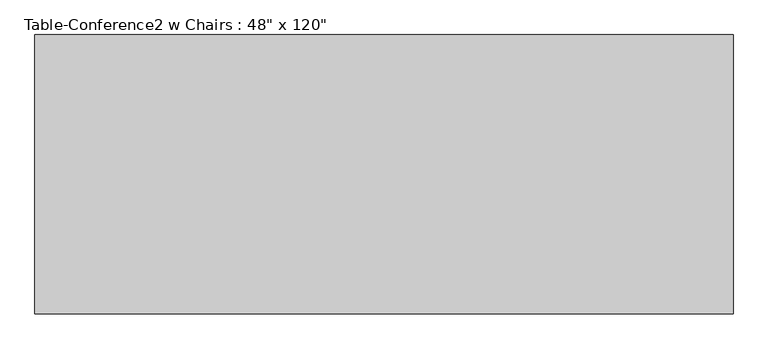
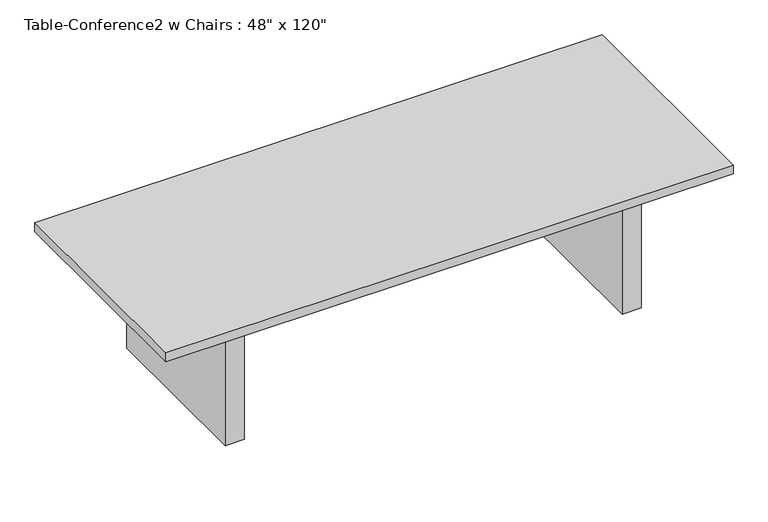
"""IFC4 building model written with IfcOpenShell, lengths in millimetres: furniture geometry."""

import ifcopenshell
import ifcopenshell.guid

model = None  # the IFC model being written
_history = None  # IfcOwnerHistory: only IFC2X3 demands one
_inside = {}  # id of a spatial element -> (the spatial element, [elements in it])
_under = {}  # id of a project, library or spatial element -> (it, [spatial elements below it])
_declared = {}  # id of a project -> (the project, [libraries it declares])
_typed = {}  # id of a type object -> (the type object, [elements of that type])
_made_of = {}  # id of a material, layer set ... -> (it, [elements and type objects made of it])


def new_model(schema):
    """Start an empty IFC model of exactly this schema.

    Asked for "IFC4X3", IfcOpenShell would pick the latest addendum, in which some entities
    have other attributes; the version numbers below select the first issue.
    IFC2X3 requires an IfcOwnerHistory on every rooted entity: one is made here for all.
    """
    global model, _history
    if schema == "IFC4X3":
        model = ifcopenshell.file(schema_version=(4, 3, 0, 0))
    else:
        model = ifcopenshell.file(schema=schema)
    _inside.clear()
    _under.clear()
    _declared.clear()
    _typed.clear()
    _made_of.clear()
    _history = None
    if model.schema == "IFC2X3":
        org = make("IfcOrganization", Name="unknown")
        user = make(
            "IfcPersonAndOrganization",
            ThePerson=make("IfcPerson", FamilyName="unknown"),
            TheOrganization=org,
        )
        app = make(
            "IfcApplication",
            ApplicationDeveloper=org,
            Version="unknown",
            ApplicationFullName="unknown",
            ApplicationIdentifier="unknown",
        )
        _history = make(
            "IfcOwnerHistory",
            OwningUser=user,
            OwningApplication=app,
            ChangeAction="ADDED",
            CreationDate=0,
        )
    return model


def make(cls, **values):
    """One entity of the class cls with the attributes given. An attribute that is None is left unset."""
    return model.create_entity(
        cls, **{name: value for name, value in values.items() if value is not None}
    )


def rooted(cls, **values):
    """An entity with a GlobalId (a new one), such as an element, a storey or a relation."""
    return make(cls, GlobalId=ifcopenshell.guid.new(), OwnerHistory=_history, **values)


def si_unit(unit_type, name, prefix=None):
    """IfcSIUnit, for example si_unit("LENGTHUNIT", "METRE", prefix="MILLI")."""
    return make("IfcSIUnit", UnitType=unit_type, Prefix=prefix, Name=name)


def assignment(units):
    """IfcUnitAssignment: the units of a project."""
    return None if units is None else make("IfcUnitAssignment", Units=units)


def point(xyz):
    """IfcCartesianPoint."""
    return None if xyz is None else make("IfcCartesianPoint", Coordinates=xyz)


def direction(xyz):
    """IfcDirection."""
    return None if xyz is None else make("IfcDirection", DirectionRatios=xyz)


def frame(location, z_axis=None, x_axis=None):
    """IfcAxis2Placement3D, a coordinate frame: its origin and axes. An axis left out is left unset."""
    return make(
        "IfcAxis2Placement3D",
        Location=point(location),
        Axis=direction(z_axis),
        RefDirection=direction(x_axis),
    )


def origin():
    """The frame at (0, 0, 0) with its axes left unset."""
    return frame((0.0, 0.0, 0.0))


def origin_with_axes():
    """The frame at (0, 0, 0) with the z axis (0, 0, 1) and the x axis (1, 0, 0) written out."""
    return frame((0.0, 0.0, 0.0), z_axis=(0.0, 0.0, 1.0), x_axis=(1.0, 0.0, 0.0))


def place(relative_to, where):
    """IfcLocalPlacement: puts the frame where relative to a parent placement (None: the world)."""
    return make(
        "IfcLocalPlacement", PlacementRelTo=relative_to, RelativePlacement=where
    )


def context(
    kind, dimensions, precision=None, world=None, true_north=None, identifier=None
):
    """IfcGeometricRepresentationContext, for example the 3D "Model" context."""
    return make(
        "IfcGeometricRepresentationContext",
        ContextIdentifier=identifier,
        ContextType=kind,
        CoordinateSpaceDimension=dimensions,
        Precision=precision,
        WorldCoordinateSystem=world,
        TrueNorth=true_north,
    )


def project(units=None, contexts=None):
    """IfcProject with its units and contexts."""
    return rooted(
        "IfcProject",
        Name="project",
        RepresentationContexts=contexts,
        UnitsInContext=assignment(units),
    )


def spatial(cls, under=None, at=None, **own):
    """A site, building, storey or space (cls), placed at a placement, below another one or the project."""
    s = rooted(cls, ObjectPlacement=at, **own)
    if under is not None:
        _under.setdefault(under.id(), (under, []))[1].append(s)
    return s


def polyline(points):
    """IfcPolyline through the points."""
    return make("IfcPolyline", Points=[point(p) for p in points])


def outline(outer, holes=None, kind="AREA"):
    """IfcArbitraryClosedProfileDef: a profile drawn as a closed curve; with holes, ...WithVoids."""
    if holes is None:
        return make("IfcArbitraryClosedProfileDef", ProfileType=kind, OuterCurve=outer)
    return make(
        "IfcArbitraryProfileDefWithVoids",
        ProfileType=kind,
        OuterCurve=outer,
        InnerCurves=holes,
    )


def extrude(swept, where, along, depth):
    """IfcExtrudedAreaSolid: the profile swept, set in the frame where, extruded along a direction by depth."""
    return make(
        "IfcExtrudedAreaSolid",
        SweptArea=swept,
        Position=where,
        ExtrudedDirection=direction(along),
        Depth=depth,
    )


def shape(context_of_items, identifier, shape_type, items):
    """IfcShapeRepresentation: the items that make up one representation, for example the "Body"."""
    return make(
        "IfcShapeRepresentation",
        ContextOfItems=context_of_items,
        RepresentationIdentifier=identifier,
        RepresentationType=shape_type,
        Items=items,
    )


def source(mapping_origin, context_of_items, identifier, shape_type, items):
    """IfcRepresentationMap: a shape defined once, which mapped items show again and again."""
    return make(
        "IfcRepresentationMap",
        MappingOrigin=mapping_origin,
        MappedRepresentation=shape(context_of_items, identifier, shape_type, items),
    )


def transform(
    local_origin,
    x_axis=None,
    y_axis=None,
    z_axis=None,
    scale=None,
    scale2=None,
    scale3=None,
    uniform=True,
):
    """IfcCartesianTransformationOperator3D, or its non-uniform kind. x_axis, y_axis, z_axis: its Axis1, 2, 3."""
    if uniform:
        return make(
            "IfcCartesianTransformationOperator3D",
            Axis1=direction(x_axis),
            Axis2=direction(y_axis),
            LocalOrigin=point(local_origin),
            Scale=scale,
            Axis3=direction(z_axis),
        )
    return make(
        "IfcCartesianTransformationOperator3DnonUniform",
        Axis1=direction(x_axis),
        Axis2=direction(y_axis),
        LocalOrigin=point(local_origin),
        Scale=scale,
        Axis3=direction(z_axis),
        Scale2=scale2,
        Scale3=scale3,
    )


def mapped(mapping_source, mapping_target):
    """IfcMappedItem: shows the shape of a source again, moved by a transform."""
    return make(
        "IfcMappedItem", MappingSource=mapping_source, MappingTarget=mapping_target
    )


def made_of(thing, what):
    """Note that an element or type object is made of a material, layer set ...; save() writes the relation."""
    if what is not None:
        _made_of.setdefault(what.id(), (what, []))[1].append(thing)
    return thing


def element(
    cls,
    number,
    at=None,
    inside=None,
    cuts=None,
    type_object=None,
    material=None,
    context=None,
    identifier="Body",
    shape_type=None,
    held_by="IfcProductDefinitionShape",
    body=None,
    shapes=None,
    **own,
):
    """One element of the class cls, such as IfcWall. Its Tag is "e" and its number.

    at: its placement. inside: the storey or other place that contains it. cuts: it is an
    opening in that element (IfcRelVoidsElement). A single representation is given by context,
    identifier, shape_type and body (its items); several are given by shapes. held_by: the class
    of the entity that holds the representations. save() writes the other relations.
    """
    e = rooted(cls, Tag="e%d" % number, ObjectPlacement=at, **own)
    if body is not None:
        shapes = [shape(context, identifier, shape_type, body)]
    if shapes is not None:
        e.Representation = make(held_by, Representations=shapes)
    if inside is not None:
        _inside.setdefault(inside.id(), (inside, []))[1].append(e)
    if cuts is not None:
        rooted(
            "IfcRelVoidsElement", RelatingBuildingElement=cuts, RelatedOpeningElement=e
        )
    if type_object is not None:
        _typed.setdefault(type_object.id(), (type_object, []))[1].append(e)
    return made_of(e, material)


def aggregate(whole, parts):
    """IfcRelAggregates: a whole, such as a stair, and the parts it consists of."""
    return rooted("IfcRelAggregates", RelatingObject=whole, RelatedObjects=parts)


def save(model, path):
    """Write the relations noted so far, then the file.

    IfcRelAggregates (storeys below a building ...), IfcRelContainedInSpatialStructure (elements
    in a storey), IfcRelDefinesByType, IfcRelAssociatesMaterial and IfcRelDeclares: one each for
    every whole, place, type object, material and project.
    """
    for whole, parts in _under.values():
        aggregate(whole, parts)
    for where, things in _inside.values():
        rooted(
            "IfcRelContainedInSpatialStructure",
            RelatedElements=things,
            RelatingStructure=where,
        )
    for kind, things in _typed.values():
        rooted("IfcRelDefinesByType", RelatedObjects=things, RelatingType=kind)
    for what, things in _made_of.values():
        rooted("IfcRelAssociatesMaterial", RelatedObjects=things, RelatingMaterial=what)
    for by, libraries in _declared.values():
        rooted("IfcRelDeclares", RelatingContext=by, RelatedDefinitions=libraries)
    model.write(path)


def furniture_098dae9e(model_context):
    return source(origin(), model_context, "Body", "SweptSolid", [
        extrude(outline(polyline([(1016.0, 457.2), (1016.0, 419.1), (-1016.0, 419.1), (-1016.0, 457.2), (1016.0, 457.2)])), frame((0.0, 0.0, 609.6), z_axis=(0.0, 0.0, 1.0), x_axis=(1.0, 0.0, 0.0)), (0.0, 0.0, 1.0), 101.6),
        extrude(outline(polyline([(1016.0, -457.2), (-1016.0, -457.2), (-1016.0, -419.1), (1016.0, -419.1), (1016.0, -457.2)])), frame((0.0, 0.0, 609.6), z_axis=(0.0, 0.0, 1.0), x_axis=(1.0, 0.0, 0.0)), (0.0, 0.0, 1.0), 101.6),
        extrude(outline(polyline([(-1016.0, -457.2), (-1117.6, -457.2), (-1117.6, 457.2), (-1016.0, 457.2), (-1016.0, -457.2)])), origin_with_axes(), (0.0, 0.0, 1.0), 711.2),
        extrude(outline(polyline([(1117.6, -457.2), (1016.0, -457.2), (1016.0, 457.2), (1117.6, 457.2), (1117.6, -457.2)])), origin_with_axes(), (0.0, 0.0, 1.0), 711.2),
        extrude(outline(polyline([(1524.0, -609.6), (-1524.0, -609.6), (-1524.0, 609.6), (1524.0, 609.6), (1524.0, -609.6)])), frame((0.0, 0.0, 711.2), z_axis=(0.0, 0.0, 1.0), x_axis=(1.0, 0.0, 0.0)), (0.0, 0.0, 1.0), 50.8),
    ])


if __name__ == "__main__":
    model = new_model("IFC4")
    model_context = context("Model", 3, world=origin())
    ifc_project = project(units=[si_unit("LENGTHUNIT", "METRE", prefix="MILLI")], contexts=[model_context])
    site = spatial("IfcSite", under=ifc_project)
    building = spatial("IfcBuilding", under=site)
    placement = place(None, origin())
    furniture_shape = furniture_098dae9e(model_context)
    element("IfcFurniture", 1, ObjectType="Table-Conference2 w Chairs : 48\" x 120\"", at=placement, inside=building, context=model_context, shape_type="MappedRepresentation", body=[
        mapped(furniture_shape, transform((0.0, 0.0, 0.0), x_axis=(1.0, 0.0, 0.0), y_axis=(0.0, 1.0, 0.0), z_axis=(0.0, 0.0, 1.0))),
    ])
    save(model, "model.ifc")

# Revit data of these elements
# Project information
#   Projekt-Nummer = "Hier die Projektnummer eintragen!"
#   IfcSite GUID = "3DdyCULLv3kQRx$MQ8PThJ"
#   IfcBuilding GUID = "3DdyCULLv3kQRx$MQ8PThG"
#   IfcProject GUID = "3DdyCULLv3kQRx$MQ8PThH"
#   Classification.Facility.Number = "Co_20_15_58"
#   Classification.Facility.Description = "Office complexes"
#   Project Status = "Projektstatus"
#   Project Address = "Geben Sie die Adresse hier ein"
# Type "Table-Conference2 w Chairs : 48\" x 120\""
#   Type IfcGUID = "2u0XNFrAPALBFZCv81fqig"
#   Assembly Code = "E2020200"
#   Description = "Seating 10-12"
#   Height = 0.762 m
#   Length = 3.048 m
#   Width = 1.2192 m
#   Number Of Chairs One Side = 4
#   Number Of Chairs = 10
#   Material = Wood - Cherry
#   Default Elevation = 0
# Element 1 (IfcFurniture, "Table-Conference2 w Chairs : 48\" x 120\"")
#   Materials on its faces: "Wood - Cherry"
# Materials
#   "Wood - Cherry": class "Wood", colour RGB 226 177 128, transparency 0
